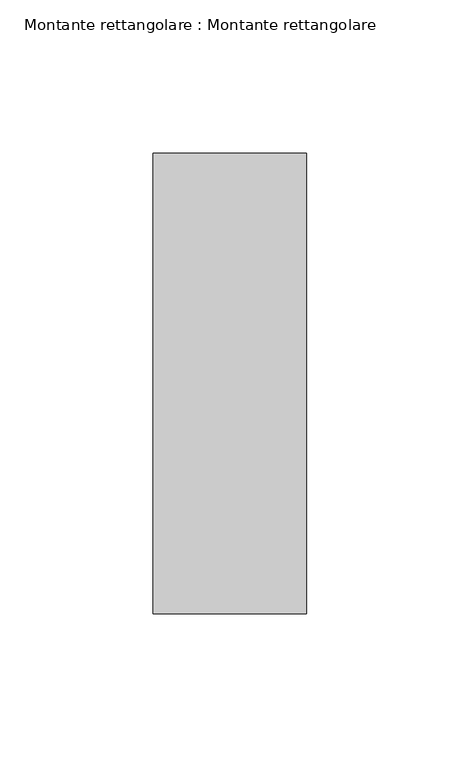
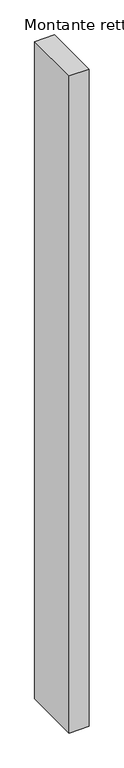
"""IFC4 building model written with IfcOpenShell, lengths in millimetres: member geometry, Montante rettangolare : Montante rettangolare."""

from ifc_helpers import new_model, si_unit, frame, origin, place, context, project, spatial, polyline, outline, extrude, source, transform, mapped, element, save


def montante_rettangolare_montante_rettangolare_b878ced1(model_context):
    return source(origin(), model_context, "Body", "SweptSolid", [
        extrude(outline(polyline([(0.0, 75.0), (0.0, -75.0), (-50.0, -75.0), (-50.0, 75.0), (0.0, 75.0)])), frame((0.0, 0.0, -1745.0), z_axis=(0.0, 0.0, 1.0), x_axis=(1.0, 0.0, 0.0)), (0.0, 0.0, 1.0), 1745.0),
    ])


if __name__ == "__main__":
    model = new_model("IFC4")
    model_context = context("Model", 3, world=origin())
    ifc_project = project(units=[si_unit("LENGTHUNIT", "METRE", prefix="MILLI")], contexts=[model_context])
    site = spatial("IfcSite", under=ifc_project)
    building = spatial("IfcBuilding", under=site)
    placement = place(None, origin())
    montante_rettangolare_montante_rettangolare_shape = montante_rettangolare_montante_rettangolare_b878ced1(model_context)
    element("IfcMember", 1, ObjectType="Montante rettangolare : Montante rettangolare", at=placement, inside=building, context=model_context, shape_type="MappedRepresentation", body=[
        mapped(montante_rettangolare_montante_rettangolare_shape, transform((0.0, 0.0, 0.0), x_axis=(1.0, 0.0, 0.0), y_axis=(0.0, 1.0, 0.0), z_axis=(0.0, 0.0, 1.0))),
    ])
    save(model, "model.ifc")

# Revit data of these elements
# Type "Montante rettangolare : Montante rettangolare"
#   built-in parameter 1007304 = 0.492126 (stored number, unit not read)
#   built-in parameter 1007301 = 0.082021 (stored number, unit not read)
#   built-in parameter 1007300 = 0.082021 (stored number, unit not read)
# Element 1 (IfcMember, "Montante rettangolare : Montante rettangolare")
#   Materials on its faces: "Acciaio"
# Materials
#   "Acciaio": class "Metallo", colour RGB 247 247 247, transparency 0, Description = "Acciaio, finitura zigrinata", Cost = 0
